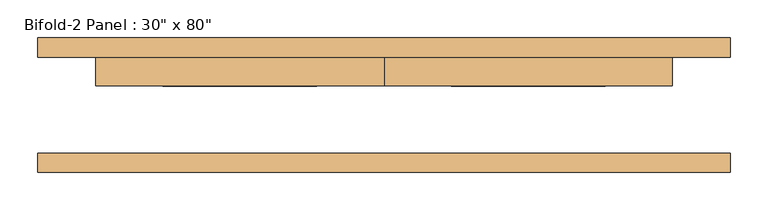
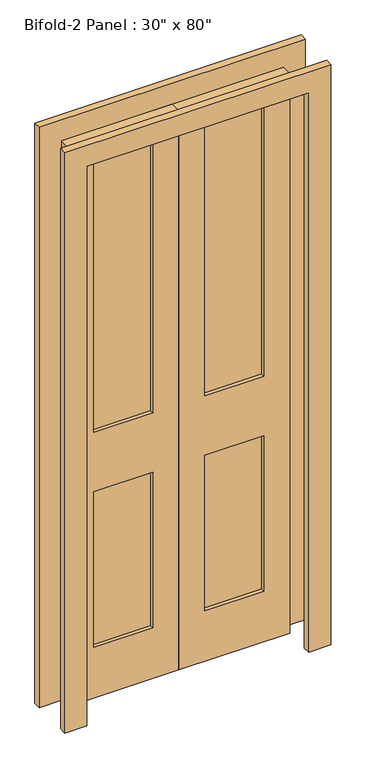
"""IFC4 building model written with IfcOpenShell, lengths in millimetres: door geometry."""

import ifcopenshell
import ifcopenshell.guid

model = None  # the IFC model being written
_history = None  # IfcOwnerHistory: only IFC2X3 demands one
_inside = {}  # id of a spatial element -> (the spatial element, [elements in it])
_under = {}  # id of a project, library or spatial element -> (it, [spatial elements below it])
_declared = {}  # id of a project -> (the project, [libraries it declares])
_typed = {}  # id of a type object -> (the type object, [elements of that type])
_made_of = {}  # id of a material, layer set ... -> (it, [elements and type objects made of it])


def new_model(schema):
    """Start an empty IFC model of exactly this schema.

    Asked for "IFC4X3", IfcOpenShell would pick the latest addendum, in which some entities
    have other attributes; the version numbers below select the first issue.
    IFC2X3 requires an IfcOwnerHistory on every rooted entity: one is made here for all.
    """
    global model, _history
    if schema == "IFC4X3":
        model = ifcopenshell.file(schema_version=(4, 3, 0, 0))
    else:
        model = ifcopenshell.file(schema=schema)
    _inside.clear()
    _under.clear()
    _declared.clear()
    _typed.clear()
    _made_of.clear()
    _history = None
    if model.schema == "IFC2X3":
        org = make("IfcOrganization", Name="unknown")
        user = make(
            "IfcPersonAndOrganization",
            ThePerson=make("IfcPerson", FamilyName="unknown"),
            TheOrganization=org,
        )
        app = make(
            "IfcApplication",
            ApplicationDeveloper=org,
            Version="unknown",
            ApplicationFullName="unknown",
            ApplicationIdentifier="unknown",
        )
        _history = make(
            "IfcOwnerHistory",
            OwningUser=user,
            OwningApplication=app,
            ChangeAction="ADDED",
            CreationDate=0,
        )
    return model


def make(cls, **values):
    """One entity of the class cls with the attributes given. An attribute that is None is left unset."""
    return model.create_entity(
        cls, **{name: value for name, value in values.items() if value is not None}
    )


def rooted(cls, **values):
    """An entity with a GlobalId (a new one), such as an element, a storey or a relation."""
    return make(cls, GlobalId=ifcopenshell.guid.new(), OwnerHistory=_history, **values)


def si_unit(unit_type, name, prefix=None):
    """IfcSIUnit, for example si_unit("LENGTHUNIT", "METRE", prefix="MILLI")."""
    return make("IfcSIUnit", UnitType=unit_type, Prefix=prefix, Name=name)


def assignment(units):
    """IfcUnitAssignment: the units of a project."""
    return None if units is None else make("IfcUnitAssignment", Units=units)


def point(xyz):
    """IfcCartesianPoint."""
    return None if xyz is None else make("IfcCartesianPoint", Coordinates=xyz)


def direction(xyz):
    """IfcDirection."""
    return None if xyz is None else make("IfcDirection", DirectionRatios=xyz)


def frame(location, z_axis=None, x_axis=None):
    """IfcAxis2Placement3D, a coordinate frame: its origin and axes. An axis left out is left unset."""
    return make(
        "IfcAxis2Placement3D",
        Location=point(location),
        Axis=direction(z_axis),
        RefDirection=direction(x_axis),
    )


def origin():
    """The frame at (0, 0, 0) with its axes left unset."""
    return frame((0.0, 0.0, 0.0))


def place(relative_to, where):
    """IfcLocalPlacement: puts the frame where relative to a parent placement (None: the world)."""
    return make(
        "IfcLocalPlacement", PlacementRelTo=relative_to, RelativePlacement=where
    )


def context(
    kind, dimensions, precision=None, world=None, true_north=None, identifier=None
):
    """IfcGeometricRepresentationContext, for example the 3D "Model" context."""
    return make(
        "IfcGeometricRepresentationContext",
        ContextIdentifier=identifier,
        ContextType=kind,
        CoordinateSpaceDimension=dimensions,
        Precision=precision,
        WorldCoordinateSystem=world,
        TrueNorth=true_north,
    )


def project(units=None, contexts=None):
    """IfcProject with its units and contexts."""
    return rooted(
        "IfcProject",
        Name="project",
        RepresentationContexts=contexts,
        UnitsInContext=assignment(units),
    )


def spatial(cls, under=None, at=None, **own):
    """A site, building, storey or space (cls), placed at a placement, below another one or the project."""
    s = rooted(cls, ObjectPlacement=at, **own)
    if under is not None:
        _under.setdefault(under.id(), (under, []))[1].append(s)
    return s


def polyline(points):
    """IfcPolyline through the points."""
    return make("IfcPolyline", Points=[point(p) for p in points])


def outline(outer, holes=None, kind="AREA"):
    """IfcArbitraryClosedProfileDef: a profile drawn as a closed curve; with holes, ...WithVoids."""
    if holes is None:
        return make("IfcArbitraryClosedProfileDef", ProfileType=kind, OuterCurve=outer)
    return make(
        "IfcArbitraryProfileDefWithVoids",
        ProfileType=kind,
        OuterCurve=outer,
        InnerCurves=holes,
    )


def extrude(swept, where, along, depth):
    """IfcExtrudedAreaSolid: the profile swept, set in the frame where, extruded along a direction by depth."""
    return make(
        "IfcExtrudedAreaSolid",
        SweptArea=swept,
        Position=where,
        ExtrudedDirection=direction(along),
        Depth=depth,
    )


def shape(context_of_items, identifier, shape_type, items):
    """IfcShapeRepresentation: the items that make up one representation, for example the "Body"."""
    return make(
        "IfcShapeRepresentation",
        ContextOfItems=context_of_items,
        RepresentationIdentifier=identifier,
        RepresentationType=shape_type,
        Items=items,
    )


def source(mapping_origin, context_of_items, identifier, shape_type, items):
    """IfcRepresentationMap: a shape defined once, which mapped items show again and again."""
    return make(
        "IfcRepresentationMap",
        MappingOrigin=mapping_origin,
        MappedRepresentation=shape(context_of_items, identifier, shape_type, items),
    )


def transform(
    local_origin,
    x_axis=None,
    y_axis=None,
    z_axis=None,
    scale=None,
    scale2=None,
    scale3=None,
    uniform=True,
):
    """IfcCartesianTransformationOperator3D, or its non-uniform kind. x_axis, y_axis, z_axis: its Axis1, 2, 3."""
    if uniform:
        return make(
            "IfcCartesianTransformationOperator3D",
            Axis1=direction(x_axis),
            Axis2=direction(y_axis),
            LocalOrigin=point(local_origin),
            Scale=scale,
            Axis3=direction(z_axis),
        )
    return make(
        "IfcCartesianTransformationOperator3DnonUniform",
        Axis1=direction(x_axis),
        Axis2=direction(y_axis),
        LocalOrigin=point(local_origin),
        Scale=scale,
        Axis3=direction(z_axis),
        Scale2=scale2,
        Scale3=scale3,
    )


def mapped(mapping_source, mapping_target):
    """IfcMappedItem: shows the shape of a source again, moved by a transform."""
    return make(
        "IfcMappedItem", MappingSource=mapping_source, MappingTarget=mapping_target
    )


def made_of(thing, what):
    """Note that an element or type object is made of a material, layer set ...; save() writes the relation."""
    if what is not None:
        _made_of.setdefault(what.id(), (what, []))[1].append(thing)
    return thing


def element(
    cls,
    number,
    at=None,
    inside=None,
    cuts=None,
    type_object=None,
    material=None,
    context=None,
    identifier="Body",
    shape_type=None,
    held_by="IfcProductDefinitionShape",
    body=None,
    shapes=None,
    **own,
):
    """One element of the class cls, such as IfcWall. Its Tag is "e" and its number.

    at: its placement. inside: the storey or other place that contains it. cuts: it is an
    opening in that element (IfcRelVoidsElement). A single representation is given by context,
    identifier, shape_type and body (its items); several are given by shapes. held_by: the class
    of the entity that holds the representations. save() writes the other relations.
    """
    e = rooted(cls, Tag="e%d" % number, ObjectPlacement=at, **own)
    if body is not None:
        shapes = [shape(context, identifier, shape_type, body)]
    if shapes is not None:
        e.Representation = make(held_by, Representations=shapes)
    if inside is not None:
        _inside.setdefault(inside.id(), (inside, []))[1].append(e)
    if cuts is not None:
        rooted(
            "IfcRelVoidsElement", RelatingBuildingElement=cuts, RelatedOpeningElement=e
        )
    if type_object is not None:
        _typed.setdefault(type_object.id(), (type_object, []))[1].append(e)
    return made_of(e, material)


def aggregate(whole, parts):
    """IfcRelAggregates: a whole, such as a stair, and the parts it consists of."""
    return rooted("IfcRelAggregates", RelatingObject=whole, RelatedObjects=parts)


def save(model, path):
    """Write the relations noted so far, then the file.

    IfcRelAggregates (storeys below a building ...), IfcRelContainedInSpatialStructure (elements
    in a storey), IfcRelDefinesByType, IfcRelAssociatesMaterial and IfcRelDeclares: one each for
    every whole, place, type object, material and project.
    """
    for whole, parts in _under.values():
        aggregate(whole, parts)
    for where, things in _inside.values():
        rooted(
            "IfcRelContainedInSpatialStructure",
            RelatedElements=things,
            RelatingStructure=where,
        )
    for kind, things in _typed.values():
        rooted("IfcRelDefinesByType", RelatedObjects=things, RelatingType=kind)
    for what, things in _made_of.values():
        rooted("IfcRelAssociatesMaterial", RelatedObjects=things, RelatingMaterial=what)
    for by, libraries in _declared.values():
        rooted("IfcRelDeclares", RelatingContext=by, RelatedDefinitions=libraries)
    model.write(path)


def door_1a011cc6(model_context):
    return source(origin(), model_context, "Body", "SweptSolid", [
        extrude(outline(polyline([(2032.0, 0.0), (2032.0, -381.0), (0.0, -381.0), (0.0, 0.0), (2032.0, 0.0)]), holes=[polyline([(1943.1, -88.9), (965.11872, -88.9), (965.11872, -292.1), (1943.1, -292.1), (1943.1, -88.9)]), polyline([(749.3, -88.9), (184.15, -88.9), (184.15, -292.1), (749.3, -292.1), (749.3, -88.9)])]), frame((0.0, 25.4, 0.0), z_axis=(0.0, 1.0, 0.0), x_axis=(0.0, 0.0, 1.0)), (0.0, 0.0, 1.0), 38.1),
        extrude(outline(polyline([(-88.9, 38.1), (-292.1, 38.1), (-292.1, 50.8), (-88.9, 50.8), (-88.9, 38.1)])), frame((0.0, 0.0, 965.11872), z_axis=(0.0, 0.0, 1.0), x_axis=(1.0, 0.0, 0.0)), (0.0, 0.0, 1.0), 977.98128),
        extrude(outline(polyline([(-88.9, 38.1), (-292.1, 38.1), (-292.1, 50.8), (-88.9, 50.8), (-88.9, 38.1)])), frame((0.0, 0.0, 184.15), z_axis=(0.0, 0.0, 1.0), x_axis=(1.0, 0.0, 0.0)), (0.0, 0.0, 1.0), 565.15),
        extrude(outline(polyline([(292.1, 38.1), (88.9, 38.1), (88.9, 50.8), (292.1, 50.8), (292.1, 38.1)])), frame((0.0, 0.0, 965.11872), z_axis=(0.0, 0.0, 1.0), x_axis=(1.0, 0.0, 0.0)), (0.0, 0.0, 1.0), 977.98128),
        extrude(outline(polyline([(292.1, 38.1), (88.9, 38.1), (88.9, 50.8), (292.1, 50.8), (292.1, 38.1)])), frame((0.0, 0.0, 184.15), z_axis=(0.0, 0.0, 1.0), x_axis=(1.0, 0.0, 0.0)), (0.0, 0.0, 1.0), 565.15),
        extrude(outline(polyline([(2108.2, -457.2), (0.0, -457.2), (0.0, -381.0), (2032.0, -381.0), (2032.0, 381.0), (0.0, 381.0), (0.0, 457.2), (2108.2, 457.2), (2108.2, -457.2)])), frame((0.0, 63.5, 0.0), z_axis=(0.0, 1.0, 0.0), x_axis=(0.0, 0.0, 1.0)), (0.0, 0.0, 1.0), 25.4),
        extrude(outline(polyline([(2108.2, 457.2), (2108.2, -457.2), (0.0, -457.2), (0.0, -381.0), (2032.0, -381.0), (2032.0, 381.0), (0.0, 381.0), (0.0, 457.2), (2108.2, 457.2)])), frame((0.0, -88.9, 0.0), z_axis=(0.0, 1.0, 0.0), x_axis=(0.0, 0.0, 1.0)), (0.0, 0.0, 1.0), 25.4),
        extrude(outline(polyline([(2032.0, 381.0), (2032.0, 0.0), (0.0, 0.0), (0.0, 381.0), (2032.0, 381.0)]), holes=[polyline([(1943.1, 88.9), (1943.1, 292.1), (965.11872, 292.1), (965.11872, 88.9), (1943.1, 88.9)]), polyline([(749.3, 88.9), (749.3, 292.1), (184.15, 292.1), (184.15, 88.9), (749.3, 88.9)])]), frame((0.0, 25.4, 0.0), z_axis=(0.0, 1.0, 0.0), x_axis=(0.0, 0.0, 1.0)), (0.0, 0.0, 1.0), 38.1),
    ])


if __name__ == "__main__":
    model = new_model("IFC4")
    model_context = context("Model", 3, world=origin())
    ifc_project = project(units=[si_unit("LENGTHUNIT", "METRE", prefix="MILLI")], contexts=[model_context])
    site = spatial("IfcSite", under=ifc_project)
    building = spatial("IfcBuilding", under=site)
    placement = place(None, origin())
    door_shape = door_1a011cc6(model_context)
    element("IfcDoor", 1, ObjectType="Bifold-2 Panel : 30\" x 80\"", at=placement, inside=building, context=model_context, shape_type="MappedRepresentation", body=[
        mapped(door_shape, transform((0.0, 0.0, 0.0), x_axis=(1.0, 0.0, 0.0), y_axis=(0.0, 1.0, 0.0), z_axis=(0.0, 0.0, 1.0))),
    ])
    save(model, "model.ifc")

# Revit data of these elements
# Type "Bifold-2 Panel : 30\" x 80\""
#   Type Mark = "11"
#   Construction Type Id = "MDOOR"
#   Assembly Code = "C1020"
#   Analytic Construction = "Metal"
#   Thickness = 0' - 1 1/2"
#   Thermal Resistance (R) = 1.5338 (h·ft²·°F)/BTU
#   Heat Transfer Coefficient (U) = 0.651978 BTU/(h·ft²·°F)
#   Height = 6' - 8"
#   Trim Projection Ext = 0' - 1"
#   Trim Projection Int = 0' - 1"
#   Trim Width = 0' - 3"
#   Width = 2' - 6"
#   Define Thermal Properties by = 1
#   Door Material = Door - Panel
#   Frame Material = Door - Frame
#   Visual Light Transmittance = 0
#   Solar Heat Gain Coefficient = 0
#   Function = (empty or 0)
#   Wall Closure = (empty or 0)
# Element 1 (IfcDoor, "Bifold-2 Panel : 30\" x 80\"")
#   Materials on its faces: "Door - Panel", "Door - Frame"
# Materials
#   "Door - Panel": class "Wood", colour RGB 210 159 95, transparency 0, Cost = 0
#   "Door - Frame": class "Miscellaneous", colour RGB 118 70 51, transparency 0, Cost = 0
